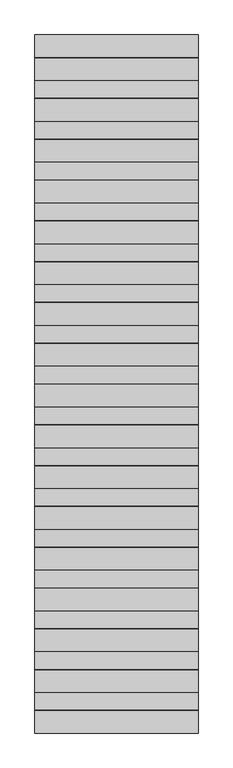
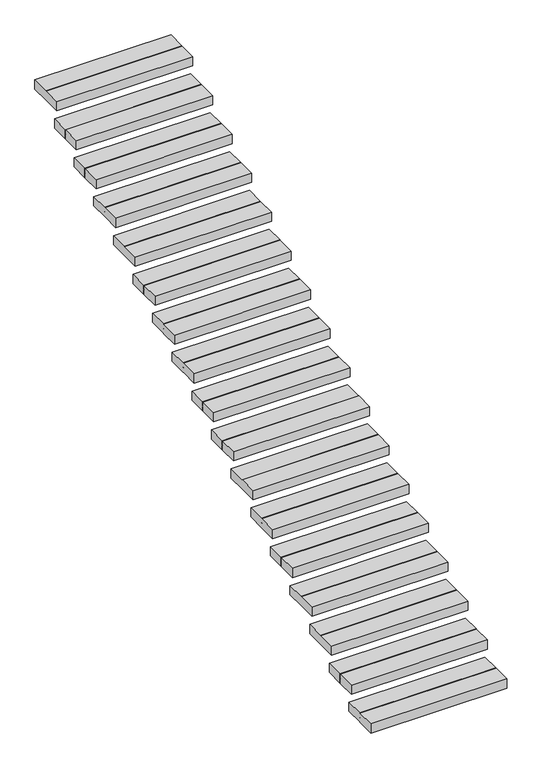
"""IFC4 building model written with IfcOpenShell, lengths in millimetres: stair flight geometry."""

from ifc_helpers import new_model, si_unit, frame, origin, place, context, project, spatial, polyline, outline, extrude, source, transform, mapped, element, save


def stair_flight_03514097(model_context):
    return source(origin(), model_context, "Body", "SweptSolid", [
        extrude(outline(polyline([(30630.8168167, 266553.7632353), (30630.8168167, 266517.2507353), (30637.1668167, 266517.2507353), (30637.1668167, 266553.7632353), (30789.5668167, 266553.7632353), (30789.5668167, 266474.3882353), (30637.1668167, 266474.3882353), (30637.1668167, 266510.9007353), (30630.8168167, 266510.9007353), (30630.8168167, 266474.3882353), (30478.4168167, 266474.3882353), (30478.4168167, 266553.7632353), (30630.8168167, 266553.7632353)])), frame((32183.3840778, 0.0, 0.0), z_axis=(1.0, 0.0, 0.0), x_axis=(0.0, 1.0, 0.0)), (0.0, 0.0, 1.0), 1117.6),
        extrude(outline(polyline([(30910.2168167, 266721.8514706), (30910.2168167, 266685.3389706), (30916.5668167, 266685.3389706), (30916.5668167, 266721.8514706), (31068.9668167, 266721.8514706), (31068.9668167, 266642.4764706), (30916.5668167, 266642.4764706), (30916.5668167, 266678.9889706), (30910.2168167, 266678.9889706), (30910.2168167, 266642.4764706), (30757.8168167, 266642.4764706), (30757.8168167, 266721.8514706), (30910.2168167, 266721.8514706)])), frame((32183.3840778, 0.0, 0.0), z_axis=(1.0, 0.0, 0.0), x_axis=(0.0, 1.0, 0.0)), (0.0, 0.0, 1.0), 1117.6),
        extrude(outline(polyline([(31189.6168167, 266889.9397059), (31189.6168167, 266853.4272059), (31195.9668167, 266853.4272059), (31195.9668167, 266889.9397059), (31348.3668167, 266889.9397059), (31348.3668167, 266810.5647059), (31195.9668167, 266810.5647059), (31195.9668167, 266847.0772059), (31189.6168167, 266847.0772059), (31189.6168167, 266810.5647059), (31037.2168167, 266810.5647059), (31037.2168167, 266889.9397059), (31189.6168167, 266889.9397059)])), frame((32183.3840778, 0.0, 0.0), z_axis=(1.0, 0.0, 0.0), x_axis=(0.0, 1.0, 0.0)), (0.0, 0.0, 1.0), 1117.6),
        extrude(outline(polyline([(31469.0168167, 267058.0279412), (31469.0168167, 267021.5154412), (31475.3668167, 267021.5154412), (31475.3668167, 267058.0279412), (31627.7668167, 267058.0279412), (31627.7668167, 266978.6529412), (31475.3668167, 266978.6529412), (31475.3668167, 267015.1654412), (31469.0168167, 267015.1654412), (31469.0168167, 266978.6529412), (31316.6168167, 266978.6529412), (31316.6168167, 267058.0279412), (31469.0168167, 267058.0279412)])), frame((32183.3840778, 0.0, 0.0), z_axis=(1.0, 0.0, 0.0), x_axis=(0.0, 1.0, 0.0)), (0.0, 0.0, 1.0), 1117.6),
        extrude(outline(polyline([(31748.4168167, 267226.1161765), (31748.4168167, 267189.6036765), (31754.7668167, 267189.6036765), (31754.7668167, 267226.1161765), (31907.1668167, 267226.1161765), (31907.1668167, 267146.7411765), (31754.7668167, 267146.7411765), (31754.7668167, 267183.2536765), (31748.4168167, 267183.2536765), (31748.4168167, 267146.7411765), (31596.0168167, 267146.7411765), (31596.0168167, 267226.1161765), (31748.4168167, 267226.1161765)])), frame((32183.3840778, 0.0, 0.0), z_axis=(1.0, 0.0, 0.0), x_axis=(0.0, 1.0, 0.0)), (0.0, 0.0, 1.0), 1117.6),
        extrude(outline(polyline([(32027.8168167, 267394.2044118), (32027.8168167, 267357.6919118), (32034.1668167, 267357.6919118), (32034.1668167, 267394.2044118), (32186.5668167, 267394.2044118), (32186.5668167, 267314.8294118), (32034.1668167, 267314.8294118), (32034.1668167, 267351.3419118), (32027.8168167, 267351.3419118), (32027.8168167, 267314.8294118), (31875.4168167, 267314.8294118), (31875.4168167, 267394.2044118), (32027.8168167, 267394.2044118)])), frame((32183.3840778, 0.0, 0.0), z_axis=(1.0, 0.0, 0.0), x_axis=(0.0, 1.0, 0.0)), (0.0, 0.0, 1.0), 1117.6),
        extrude(outline(polyline([(32307.2168167, 267562.2926471), (32307.2168167, 267525.7801471), (32313.5668167, 267525.7801471), (32313.5668167, 267562.2926471), (32465.9668167, 267562.2926471), (32465.9668167, 267482.9176471), (32313.5668167, 267482.9176471), (32313.5668167, 267519.4301471), (32307.2168167, 267519.4301471), (32307.2168167, 267482.9176471), (32154.8168167, 267482.9176471), (32154.8168167, 267562.2926471), (32307.2168167, 267562.2926471)])), frame((32183.3840778, 0.0, 0.0), z_axis=(1.0, 0.0, 0.0), x_axis=(0.0, 1.0, 0.0)), (0.0, 0.0, 1.0), 1117.6),
        extrude(outline(polyline([(32586.6168167, 267730.3808824), (32586.6168167, 267693.8683824), (32592.9668167, 267693.8683824), (32592.9668167, 267730.3808824), (32745.3668167, 267730.3808824), (32745.3668167, 267651.0058824), (32592.9668167, 267651.0058824), (32592.9668167, 267687.5183824), (32586.6168167, 267687.5183824), (32586.6168167, 267651.0058824), (32434.2168167, 267651.0058824), (32434.2168167, 267730.3808824), (32586.6168167, 267730.3808824)])), frame((32183.3840778, 0.0, 0.0), z_axis=(1.0, 0.0, 0.0), x_axis=(0.0, 1.0, 0.0)), (0.0, 0.0, 1.0), 1117.6),
        extrude(outline(polyline([(32866.0168167, 267898.4691176), (32866.0168167, 267861.9566176), (32872.3668167, 267861.9566176), (32872.3668167, 267898.4691176), (33024.7668167, 267898.4691176), (33024.7668167, 267819.0941176), (32872.3668167, 267819.0941176), (32872.3668167, 267855.6066176), (32866.0168167, 267855.6066176), (32866.0168167, 267819.0941176), (32713.6168167, 267819.0941176), (32713.6168167, 267898.4691176), (32866.0168167, 267898.4691176)])), frame((32183.3840778, 0.0, 0.0), z_axis=(1.0, 0.0, 0.0), x_axis=(0.0, 1.0, 0.0)), (0.0, 0.0, 1.0), 1117.6),
        extrude(outline(polyline([(33145.4168167, 268066.5573529), (33145.4168167, 268030.0448529), (33151.7668167, 268030.0448529), (33151.7668167, 268066.5573529), (33304.1668167, 268066.5573529), (33304.1668167, 267987.1823529), (33151.7668167, 267987.1823529), (33151.7668167, 268023.6948529), (33145.4168167, 268023.6948529), (33145.4168167, 267987.1823529), (32993.0168167, 267987.1823529), (32993.0168167, 268066.5573529), (33145.4168167, 268066.5573529)])), frame((32183.3840778, 0.0, 0.0), z_axis=(1.0, 0.0, 0.0), x_axis=(0.0, 1.0, 0.0)), (0.0, 0.0, 1.0), 1117.6),
        extrude(outline(polyline([(33424.8168167, 268234.6455882), (33424.8168167, 268198.1330882), (33431.1668167, 268198.1330882), (33431.1668167, 268234.6455882), (33583.5668167, 268234.6455882), (33583.5668167, 268155.2705882), (33431.1668167, 268155.2705882), (33431.1668167, 268191.7830882), (33424.8168167, 268191.7830882), (33424.8168167, 268155.2705882), (33272.4168167, 268155.2705882), (33272.4168167, 268234.6455882), (33424.8168167, 268234.6455882)])), frame((32183.3840778, 0.0, 0.0), z_axis=(1.0, 0.0, 0.0), x_axis=(0.0, 1.0, 0.0)), (0.0, 0.0, 1.0), 1117.6),
        extrude(outline(polyline([(33704.2168167, 268402.7338235), (33704.2168167, 268366.2213235), (33710.5668167, 268366.2213235), (33710.5668167, 268402.7338235), (33862.9668167, 268402.7338235), (33862.9668167, 268323.3588235), (33710.5668167, 268323.3588235), (33710.5668167, 268359.8713235), (33704.2168167, 268359.8713235), (33704.2168167, 268323.3588235), (33551.8168167, 268323.3588235), (33551.8168167, 268402.7338235), (33704.2168167, 268402.7338235)])), frame((32183.3840778, 0.0, 0.0), z_axis=(1.0, 0.0, 0.0), x_axis=(0.0, 1.0, 0.0)), (0.0, 0.0, 1.0), 1117.6),
        extrude(outline(polyline([(33983.6168167, 268570.8220588), (33983.6168167, 268534.3095588), (33989.9668167, 268534.3095588), (33989.9668167, 268570.8220588), (34142.3668167, 268570.8220588), (34142.3668167, 268491.4470588), (33989.9668167, 268491.4470588), (33989.9668167, 268527.9595588), (33983.6168167, 268527.9595588), (33983.6168167, 268491.4470588), (33831.2168167, 268491.4470588), (33831.2168167, 268570.8220588), (33983.6168167, 268570.8220588)])), frame((32183.3840778, 0.0, 0.0), z_axis=(1.0, 0.0, 0.0), x_axis=(0.0, 1.0, 0.0)), (0.0, 0.0, 1.0), 1117.6),
        extrude(outline(polyline([(34263.0168167, 268738.9102941), (34263.0168167, 268702.3977941), (34269.3668167, 268702.3977941), (34269.3668167, 268738.9102941), (34421.7668167, 268738.9102941), (34421.7668167, 268659.5352941), (34269.3668167, 268659.5352941), (34269.3668167, 268696.0477941), (34263.0168167, 268696.0477941), (34263.0168167, 268659.5352941), (34110.6168167, 268659.5352941), (34110.6168167, 268738.9102941), (34263.0168167, 268738.9102941)])), frame((32183.3840778, 0.0, 0.0), z_axis=(1.0, 0.0, 0.0), x_axis=(0.0, 1.0, 0.0)), (0.0, 0.0, 1.0), 1117.6),
        extrude(outline(polyline([(34542.4168167, 268906.9985294), (34542.4168167, 268870.4860294), (34548.7668167, 268870.4860294), (34548.7668167, 268906.9985294), (34701.1668167, 268906.9985294), (34701.1668167, 268827.6235294), (34548.7668167, 268827.6235294), (34548.7668167, 268864.1360294), (34542.4168167, 268864.1360294), (34542.4168167, 268827.6235294), (34390.0168167, 268827.6235294), (34390.0168167, 268906.9985294), (34542.4168167, 268906.9985294)])), frame((32183.3840778, 0.0, 0.0), z_axis=(1.0, 0.0, 0.0), x_axis=(0.0, 1.0, 0.0)), (0.0, 0.0, 1.0), 1117.6),
        extrude(outline(polyline([(34821.8168167, 269075.0867647), (34821.8168167, 269038.5742647), (34828.1668167, 269038.5742647), (34828.1668167, 269075.0867647), (34980.5668167, 269075.0867647), (34980.5668167, 268995.7117647), (34828.1668167, 268995.7117647), (34828.1668167, 269032.2242647), (34821.8168167, 269032.2242647), (34821.8168167, 268995.7117647), (34669.4168167, 268995.7117647), (34669.4168167, 269075.0867647), (34821.8168167, 269075.0867647)])), frame((32183.3840778, 0.0, 0.0), z_axis=(1.0, 0.0, 0.0), x_axis=(0.0, 1.0, 0.0)), (0.0, 0.0, 1.0), 1117.6),
        extrude(outline(polyline([(35101.2168167, 269243.175), (35101.2168167, 269206.6625), (35107.5668167, 269206.6625), (35107.5668167, 269243.175), (35259.9668167, 269243.175), (35259.9668167, 269163.8), (35107.5668167, 269163.8), (35107.5668167, 269200.3125), (35101.2168167, 269200.3125), (35101.2168167, 269163.8), (34948.8168167, 269163.8), (34948.8168167, 269243.175), (35101.2168167, 269243.175)])), frame((32183.3840778, 0.0, 0.0), z_axis=(1.0, 0.0, 0.0), x_axis=(0.0, 1.0, 0.0)), (0.0, 0.0, 1.0), 1117.6),
    ])


if __name__ == "__main__":
    model = new_model("IFC4")
    model_context = context("Model", 3, world=origin())
    ifc_project = project(units=[si_unit("LENGTHUNIT", "METRE", prefix="MILLI")], contexts=[model_context])
    site = spatial("IfcSite", under=ifc_project)
    building = spatial("IfcBuilding", under=site)
    placement = place(None, origin())
    stair_flight_shape = stair_flight_03514097(model_context)
    element("IfcStairFlight", 1, at=placement, inside=building, context=model_context, shape_type="MappedRepresentation", body=[
        mapped(stair_flight_shape, transform((0.0, 0.0, 0.0), x_axis=(1.0, 0.0, 0.0), y_axis=(0.0, 1.0, 0.0), z_axis=(0.0, 0.0, 1.0))),
    ])
    save(model, "model.ifc")

# Revit data of these elements
# Element 1 (IfcStairFlight)
#   Materials on its faces: "TREAD: (3) TREATED 4X4"
# Materials
#   "TREAD: (3) TREATED 4X4": class "Wood", colour RGB 164 134 123, transparency 0, Description = "Pinus Echinata", Cost = 0
